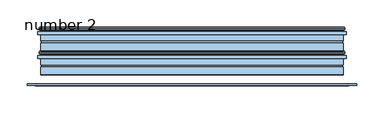
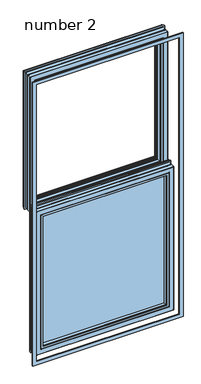
"""IFC4 building model written with IfcOpenShell, lengths in millimetres: window geometry, Window-Exterior-Sierra-Double_Hung-Operating_Unit-18inch_48inch-Width-(Hi-Divide) : number 2."""

from ifc_helpers import new_model, si_unit, frame, origin, place, context, project, spatial, polyline, ellipse_curve, outline, extrude, source, transform, mapped, element, save
from ifc_brep_helpers import plane_surface, cylinder_surface, revolved_surface, advanced_brep


def number_2_68d64fd7(model_context):
    return source(origin(), model_context, "Body", "SolidModel", [
        advanced_brep(
        [(-251.70765, 40.3779134, 2080.50765), (-251.70765, 41.5137713, 2080.50765), (251.70765, 41.5137713, 2080.50765), (251.70765, 40.3779134, 2080.50765), (-249.6812762, 41.5137713, 2078.4812762), (-249.8708265, 43.9568107, 2078.6708265), (249.8708265, 43.9568107, 2078.6708265), (249.6812762, 41.5137713, 2078.4812762), (-257.67665, 46.4921713, 2086.47665), (257.67665, 46.4921713, 2086.47665), (-257.67665, 48.8797713, 2086.47665), (257.67665, 48.8797713, 2086.47665), (-279.97785, 48.8797713, 2108.77785), (-282.36545, 46.4921713, 2111.16545), (282.36545, 46.4921713, 2111.16545), (279.97785, 48.8797713, 2108.77785), (-282.36545, 43.9267713, 2111.16545), (282.36545, 43.9267713, 2111.16545), (-280.33345, 43.9267713, 2109.13345), (-280.33345, 42.2503713, 2109.13345), (280.33345, 42.2503713, 2109.13345), (280.33345, 43.9267713, 2109.13345), (-277.03145, 42.2503713, 2105.83145), (-277.03145, 40.3453713, 2105.83145), (277.03145, 40.3453713, 2105.83145), (277.03145, 42.2503713, 2105.83145), (-284.95625, 40.3453713, 2113.75625), (-284.95625, 34.7319713, 2113.75625), (284.95625, 34.7319713, 2113.75625), (284.95625, 40.3453713, 2113.75625), (-279.64765, 34.7319713, 2108.44765), (-279.64765, 22.5399713, 2108.44765), (279.64765, 22.5399713, 2108.44765), (279.64765, 34.7319713, 2108.44765), (-279.64765, 18.5775713, 2108.44765), (279.64765, 18.5775713, 2108.44765), (-279.64765, 5.2425713, 2108.44765), (279.64765, 5.2425713, 2108.44765), (-278.83485, 4.4297713, 2107.63485), (278.83485, 4.4297713, 2107.63485), (-260.54685, 4.4297713, 2089.34685), (-260.54685, 6.3102893, 2089.34685), (260.54685, 6.3102893, 2089.34685), (260.54685, 4.4297713, 2089.34685), (-258.9459612, 6.3102893, 2087.7459612), (-258.9459612, 4.7100893, 2087.7459612), (258.9459612, 4.7100893, 2087.7459612), (258.9459612, 6.3102893, 2087.7459612), (-251.4021612, 4.7100893, 2080.2021612), (-251.4021612, 8.4780088, 2080.2021612), (251.4021612, 8.4780088, 2080.2021612), (251.4021612, 4.7100893, 2080.2021612), (-249.2398112, 8.4780088, 2078.0398112), (-248.2271612, 20.3056893, 2077.0271612), (248.2271612, 20.3056893, 2077.0271612), (249.2398112, 8.4780088, 2078.0398112), (-258.1585612, 20.3056893, 2086.9585612), (-260.54685, 17.9174005, 2089.34685), (260.54685, 17.9174005, 2089.34685), (258.1585612, 20.3056893, 2086.9585612), (-260.54685, 39.3547713, 2089.34685), (260.54685, 39.3547713, 2089.34685), (-256.9662312, 39.3547713, 2085.7662312), (-255.9430891, 40.3779134, 2084.7430891), (255.9430891, 40.3779134, 2084.7430891), (256.9662312, 39.3547713, 2085.7662312), (251.70765, 41.5137713, 1557.2486), (251.70765, 40.3779134, 1557.2486), (249.8708265, 43.9568107, 1559.0854235), (249.6812762, 41.5137713, 1559.2749738), (257.67665, 46.4921713, 1551.2796), (257.67665, 48.8797713, 1551.2796), (282.36545, 46.4921713, 1526.5908), (279.97785, 48.8797713, 1528.9784), (282.36545, 43.9267713, 1526.5908), (280.33345, 42.2503713, 1528.6228), (280.33345, 43.9267713, 1528.6228), (277.03145, 40.3453713, 1531.9248), (277.03145, 42.2503713, 1531.9248), (284.95625, 34.7319713, 1524.0), (284.95625, 40.3453713, 1524.0), (279.64765, 22.5399713, 1529.3086), (279.64765, 34.7319713, 1529.3086), (279.64765, 18.5775713, 1529.3086), (279.64765, 5.2425713, 1529.3086), (278.83485, 4.4297713, 1530.1214), (260.54685, 6.3102893, 1548.4094), (260.54685, 4.4297713, 1548.4094), (258.9459612, 4.7100893, 1550.0102888), (258.9459612, 6.3102893, 1550.0102888), (251.4021612, 8.4780088, 1557.5540888), (251.4021612, 4.7100893, 1557.5540888), (248.2271612, 20.3056893, 1560.7290888), (249.2398112, 8.4780088, 1559.7164388), (260.54685, 17.9174005, 1548.4094), (258.1585612, 20.3056893, 1550.7976888), (260.54685, 39.3547713, 1548.4094), (255.9430891, 40.3779134, 1553.0131609), (256.9662312, 39.3547713, 1551.9900188), (-251.70765, 41.5137713, 1557.2486), (-251.70765, 40.3779134, 1557.2486), (-249.8708265, 43.9568107, 1559.0854235), (-249.6812762, 41.5137713, 1559.2749738), (-257.67665, 46.4921713, 1551.2796), (-257.67665, 48.8797713, 1551.2796), (-282.36545, 46.4921713, 1526.5908), (-279.97785, 48.8797713, 1528.9784), (-282.36545, 43.9267713, 1526.5908), (-280.33345, 42.2503713, 1528.6228), (-280.33345, 43.9267713, 1528.6228), (-277.03145, 40.3453713, 1531.9248), (-277.03145, 42.2503713, 1531.9248), (-284.95625, 34.7319713, 1524.0), (-284.95625, 40.3453713, 1524.0), (-279.64765, 22.5399713, 1529.3086), (-279.64765, 34.7319713, 1529.3086), (-279.64765, 18.5775713, 1529.3086), (-279.64765, 5.2425713, 1529.3086), (-278.83485, 4.4297713, 1530.1214), (-260.54685, 6.3102893, 1548.4094), (-260.54685, 4.4297713, 1548.4094), (-258.9459612, 4.7100893, 1550.0102888), (-258.9459612, 6.3102893, 1550.0102888), (-251.4021612, 8.4780088, 1557.5540888), (-251.4021612, 4.7100893, 1557.5540888), (-248.2271612, 20.3056893, 1560.7290888), (-249.2398112, 8.4780088, 1559.7164388), (-260.54685, 17.9174005, 1548.4094), (-258.1585612, 20.3056893, 1550.7976888), (-260.54685, 39.3547713, 1548.4094), (-255.9430891, 40.3779134, 1553.0131609), (-256.9662312, 39.3547713, 1551.9900188)],
        [
            (0, 1),
            (1, 2),
            (2, 3),
            (3, 0),
            (4, 5),
            (5, 6),
            (6, 7),
            (7, 4),
            (5, 8),
            (8, 9),
            (9, 6),
            (8, 10),
            (10, 11),
            (11, 9),
            (12, 13, ellipse_curve(frame((-279.97785, 46.4921713, 2108.77785), z_axis=(0.7071067811865475, 0.0, 0.7071067811865475), x_axis=(-0.7071067811865476, 0.0, 0.7071067811865474)), 3.3765763, 2.3876)),
            (13, 14),
            (14, 15, ellipse_curve(frame((279.97785, 46.4921713, 2108.77785), z_axis=(-0.7071067811865475, 0.0, 0.7071067811865475), x_axis=(-0.7071067811865476, 0.0, -0.7071067811865474)), 3.3765763, 2.3876)),
            (15, 12),
            (13, 16),
            (16, 17),
            (17, 14),
            (18, 19),
            (19, 20),
            (20, 21),
            (21, 18),
            (22, 23),
            (23, 24),
            (24, 25),
            (25, 22),
            (26, 27),
            (27, 28),
            (28, 29),
            (29, 26),
            (30, 31),
            (31, 32),
            (32, 33),
            (33, 30),
            (31, 34, ellipse_curve(frame((-279.64765, 20.5587713, 2108.44765), z_axis=(-0.7071067811865475, 0.0, -0.7071067811865475), x_axis=(0.7071067811865476, 0.0, -0.7071067811865474)), 2.8018399, 1.9812)),
            (34, 35),
            (35, 32, ellipse_curve(frame((279.64765, 20.5587713, 2108.44765), z_axis=(0.7071067811865475, 0.0, -0.7071067811865475), x_axis=(0.7071067811865476, 0.0, 0.7071067811865474)), 2.8018399, 1.9812)),
            (34, 36),
            (36, 37),
            (37, 35),
            (36, 38, ellipse_curve(frame((-278.83485, 5.2425713, 2107.63485), z_axis=(0.7071067811865475, 0.0, 0.7071067811865475), x_axis=(-0.7071067811865476, 0.0, 0.7071067811865474)), 1.1494728, 0.8128)),
            (38, 39),
            (39, 37, ellipse_curve(frame((278.83485, 5.2425713, 2107.63485), z_axis=(-0.7071067811865475, 0.0, 0.7071067811865475), x_axis=(-0.7071067811865476, 0.0, -0.7071067811865474)), 1.1494728, 0.8128)),
            (40, 41),
            (41, 42),
            (42, 43),
            (43, 40),
            (44, 45),
            (45, 46),
            (46, 47),
            (47, 44),
            (48, 49),
            (49, 50),
            (50, 51),
            (51, 48),
            (52, 53),
            (53, 54),
            (54, 55),
            (55, 52),
            (56, 57),
            (57, 58),
            (58, 59),
            (59, 56),
            (57, 60),
            (60, 61),
            (61, 58),
            (62, 63),
            (63, 64),
            (64, 65),
            (65, 62),
            (2, 66),
            (66, 67),
            (67, 3),
            (6, 68),
            (68, 69),
            (69, 7),
            (9, 70),
            (70, 68),
            (11, 71),
            (71, 70),
            (14, 72),
            (72, 73, ellipse_curve(frame((279.97785, 46.4921713, 1528.9784), z_axis=(0.7071067811865475, 0.0, 0.7071067811865475), x_axis=(-0.7071067811865474, 0.0, 0.7071067811865476)), 3.3765763, 2.3876)),
            (73, 15),
            (17, 74),
            (74, 72),
            (20, 75),
            (75, 76),
            (76, 21),
            (24, 77),
            (77, 78),
            (78, 25),
            (28, 79),
            (79, 80),
            (80, 29),
            (32, 81),
            (81, 82),
            (82, 33),
            (35, 83),
            (83, 81, ellipse_curve(frame((279.64765, 20.5587713, 1529.3086), z_axis=(-0.7071067811865475, 0.0, -0.7071067811865475), x_axis=(0.7071067811865474, 0.0, -0.7071067811865476)), 2.8018399, 1.9812)),
            (37, 84),
            (84, 83),
            (39, 85),
            (85, 84, ellipse_curve(frame((278.83485, 5.2425713, 1530.1214), z_axis=(0.7071067811865475, 0.0, 0.7071067811865475), x_axis=(-0.7071067811865474, 0.0, 0.7071067811865476)), 1.1494728, 0.8128)),
            (42, 86),
            (86, 87),
            (87, 43),
            (46, 88),
            (88, 89),
            (89, 47),
            (50, 90),
            (90, 91),
            (91, 51),
            (54, 92),
            (92, 93),
            (93, 55),
            (58, 94),
            (94, 95),
            (95, 59),
            (61, 96),
            (96, 94),
            (64, 97),
            (97, 98),
            (98, 65),
            (66, 99),
            (99, 100),
            (100, 67),
            (68, 101),
            (101, 102),
            (102, 69),
            (70, 103),
            (103, 101),
            (71, 104),
            (104, 103),
            (72, 105),
            (105, 106, ellipse_curve(frame((-279.97785, 46.4921713, 1528.9784), z_axis=(0.7071067811865475, 0.0, -0.7071067811865475), x_axis=(0.7071067811865476, 0.0, 0.7071067811865474)), 3.3765763, 2.3876)),
            (106, 73),
            (74, 107),
            (107, 105),
            (75, 108),
            (108, 109),
            (109, 76),
            (77, 110),
            (110, 111),
            (111, 78),
            (79, 112),
            (112, 113),
            (113, 80),
            (81, 114),
            (114, 115),
            (115, 82),
            (83, 116),
            (116, 114, ellipse_curve(frame((-279.64765, 20.5587713, 1529.3086), z_axis=(-0.7071067811865475, 0.0, 0.7071067811865475), x_axis=(-0.7071067811865476, 0.0, -0.7071067811865474)), 2.8018399, 1.9812)),
            (84, 117),
            (117, 116),
            (85, 118),
            (118, 117, ellipse_curve(frame((-278.83485, 5.2425713, 1530.1214), z_axis=(0.7071067811865475, 0.0, -0.7071067811865475), x_axis=(0.7071067811865476, 0.0, 0.7071067811865474)), 1.1494728, 0.8128)),
            (86, 119),
            (119, 120),
            (120, 87),
            (88, 121),
            (121, 122),
            (122, 89),
            (90, 123),
            (123, 124),
            (124, 91),
            (92, 125),
            (125, 126),
            (126, 93),
            (94, 127),
            (127, 128),
            (128, 95),
            (96, 129),
            (129, 127),
            (97, 130),
            (130, 131),
            (131, 98),
            (63, 130),
            (100, 0),
            (99, 1),
            (102, 4),
            (101, 5),
            (103, 8),
            (104, 10),
            (106, 12),
            (105, 13),
            (107, 16),
            (109, 18),
            (108, 19),
            (111, 22),
            (110, 23),
            (113, 26),
            (112, 27),
            (115, 30),
            (114, 31),
            (116, 34),
            (117, 36),
            (118, 38),
            (120, 40),
            (119, 41),
            (122, 44),
            (121, 45),
            (124, 48),
            (123, 49),
            (126, 52),
            (125, 53),
            (128, 56),
            (127, 57),
            (129, 60),
            (131, 62),
        ],
        [
            plane_surface(frame((-251.70765, 41.5137713, 2080.50765), z_axis=(0.0, 0.0, -1.0), x_axis=(1.0, 0.0, 0.0))),
            plane_surface(frame((-249.8708265, 43.9568107, 2078.6708265), z_axis=(0.0, 0.07735544009934336, -0.9970035786731344), x_axis=(1.0, 0.0, 0.0))),
            plane_surface(frame((-257.67665, 46.4921713, 2086.47665), z_axis=(0.0, 0.9510889261909009, -0.3089172291683307), x_axis=(1.0, 0.0, 0.0))),
            plane_surface(frame((-257.67665, 48.8797713, 2086.47665), z_axis=(0.0, 0.0, -1.0), x_axis=(1.0, 0.0, 0.0))),
            cylinder_surface(frame((-284.95625, 46.4921713, 2108.77785), z_axis=(-1.0, 0.0, 0.0), x_axis=(0.0, 0.0, 1.0)), 2.3876),
            plane_surface(frame((-282.36545, 43.9267713, 2111.16545), z_axis=(0.0, 0.0, 1.0), x_axis=(1.0, 0.0, 0.0))),
            plane_surface(frame((-280.33345, 42.2503713, 2109.13345), z_axis=(0.0, 0.0, 1.0), x_axis=(1.0, 0.0, 0.0))),
            plane_surface(frame((-277.03145, 40.3453713, 2105.83145), z_axis=(0.0, 0.0, 1.0), x_axis=(1.0, 0.0, 0.0))),
            plane_surface(frame((-284.95625, 34.7319713, 2113.75625), z_axis=(0.0, 0.0, 1.0), x_axis=(1.0, 0.0, 0.0))),
            plane_surface(frame((-279.64765, 22.5399713, 2108.44765), z_axis=(0.0, 0.0, 1.0), x_axis=(1.0, 0.0, 0.0))),
            revolved_surface(polyline([(281.6288499930891, 20.5587713, 2110.4288500000002), (-281.62884999308903, 20.5587713, 2110.4288500000002)]), (-284.95625, 20.5587713, 2108.44765), (1.0, 0.0, 0.0)),
            plane_surface(frame((-279.64765, 5.2425713, 2108.44765), z_axis=(0.0, 0.0, 1.0), x_axis=(1.0, 0.0, 0.0))),
            cylinder_surface(frame((-284.95625, 5.2425713, 2107.63485), z_axis=(-1.0, 0.0, 0.0), x_axis=(0.0, 0.0, 1.0)), 0.8128),
            plane_surface(frame((-260.54685, 6.3102893, 2089.34685), z_axis=(0.0, 0.0, -1.0), x_axis=(1.0, 0.0, 0.0))),
            plane_surface(frame((-258.9459612, 4.7100893, 2087.7459612), z_axis=(0.0, 0.0, 1.0), x_axis=(1.0, 0.0, 0.0))),
            plane_surface(frame((-251.4021612, 8.4780088, 2080.2021612), z_axis=(0.0, 0.0, -1.0), x_axis=(1.0, 0.0, 0.0))),
            plane_surface(frame((-248.2271612, 20.3056893, 2077.0271612), z_axis=(0.0, -0.08530487454184653, -0.996354895797376), x_axis=(1.0, 0.0, 0.0))),
            plane_surface(frame((-260.54685, 17.9174005, 2089.34685), z_axis=(0.0, 0.7071067811865713, 0.7071067811865238), x_axis=(1.0, 0.0, 0.0))),
            plane_surface(frame((-260.54685, 39.3547713, 2089.34685), z_axis=(0.0, 0.0, -1.0), x_axis=(1.0, 0.0, 0.0))),
            plane_surface(frame((-255.9430891, 40.3779134, 2084.7430891), z_axis=(0.0, -0.7071067811861558, -0.7071067811869393), x_axis=(1.0, 0.0, 0.0))),
            plane_surface(frame((251.70765, 41.5137713, 2080.50765), z_axis=(-1.0, 0.0, 0.0), x_axis=(0.0, 0.0, -1.0))),
            plane_surface(frame((249.8708265, 43.9568107, 2078.6708265), z_axis=(-0.9970035786731344, 0.07735544009934342, 0.0), x_axis=(0.0, 0.0, -1.0))),
            plane_surface(frame((257.67665, 46.4921713, 2086.47665), z_axis=(-0.3089172291683307, 0.951088926190901, 0.0), x_axis=(0.0, 0.0, -1.0))),
            plane_surface(frame((257.67665, 48.8797713, 2086.47665), z_axis=(-1.0, 0.0, 0.0), x_axis=(0.0, 0.0, -1.0))),
            cylinder_surface(frame((279.97785, 46.4921713, 2113.75625), z_axis=(0.0, 0.0, 1.0), x_axis=(1.0, 0.0, 0.0)), 2.3876),
            plane_surface(frame((282.36545, 43.9267713, 2111.16545), z_axis=(1.0, 0.0, 0.0), x_axis=(0.0, 0.0, -1.0))),
            plane_surface(frame((280.33345, 42.2503713, 2109.13345), z_axis=(1.0, 0.0, 0.0), x_axis=(0.0, 0.0, -1.0))),
            plane_surface(frame((277.03145, 40.3453713, 2105.83145), z_axis=(1.0, 0.0, 0.0), x_axis=(0.0, 0.0, -1.0))),
            plane_surface(frame((284.95625, 34.7319713, 2113.75625), z_axis=(1.0, 0.0, 0.0), x_axis=(0.0, 0.0, -1.0))),
            plane_surface(frame((279.64765, 22.5399713, 2108.44765), z_axis=(1.0, 0.0, 0.0), x_axis=(0.0, 0.0, -1.0))),
            revolved_surface(polyline([(281.62885, 20.5587713, 1527.327400006911), (281.62885, 20.5587713, 2110.428849993089)]), (279.64765, 20.5587713, 2113.75625), (0.0, 0.0, -1.0)),
            plane_surface(frame((279.64765, 5.2425713, 2108.44765), z_axis=(1.0, 0.0, 0.0), x_axis=(0.0, 0.0, -1.0))),
            cylinder_surface(frame((278.83485, 5.2425713, 2113.75625), z_axis=(0.0, 0.0, 1.0), x_axis=(1.0, 0.0, 0.0)), 0.8128),
            plane_surface(frame((260.54685, 6.3102893, 2089.34685), z_axis=(-1.0, 0.0, 0.0), x_axis=(0.0, 0.0, -1.0))),
            plane_surface(frame((258.9459612, 4.7100893, 2087.7459612), z_axis=(1.0, 0.0, 0.0), x_axis=(0.0, 0.0, -1.0))),
            plane_surface(frame((251.4021612, 8.4780088, 2080.2021612), z_axis=(-1.0, 0.0, 0.0), x_axis=(0.0, 0.0, -1.0))),
            plane_surface(frame((248.2271612, 20.3056893, 2077.0271612), z_axis=(-0.996354895797376, -0.08530487454184647, 0.0), x_axis=(0.0, 0.0, -1.0))),
            plane_surface(frame((260.54685, 17.9174005, 2089.34685), z_axis=(0.7071067811865238, 0.7071067811865713, 0.0), x_axis=(0.0, 0.0, -1.0))),
            plane_surface(frame((260.54685, 39.3547713, 2089.34685), z_axis=(-1.0, 0.0, 0.0), x_axis=(0.0, 0.0, -1.0))),
            plane_surface(frame((255.9430891, 40.3779134, 2084.7430891), z_axis=(-0.7071067811869393, -0.7071067811861558, 0.0), x_axis=(0.0, 0.0, -1.0))),
            plane_surface(frame((251.70765, 41.5137713, 1557.2486), z_axis=(0.0, 0.0, 1.0), x_axis=(-1.0, 0.0, 0.0))),
            plane_surface(frame((249.8708265, 43.9568107, 1559.0854235), z_axis=(0.0, 0.07735544009934348, 0.9970035786731344), x_axis=(-1.0, 0.0, 0.0))),
            plane_surface(frame((257.67665, 46.4921713, 1551.2796), z_axis=(0.0, 0.951088926190901, 0.30891722916833064), x_axis=(-1.0, 0.0, 0.0))),
            plane_surface(frame((257.67665, 48.8797713, 1551.2796), z_axis=(0.0, 0.0, 1.0), x_axis=(-1.0, 0.0, 0.0))),
            cylinder_surface(frame((284.95625, 46.4921713, 1528.9784), z_axis=(1.0, 0.0, 0.0), x_axis=(0.0, 0.0, -1.0)), 2.3876),
            plane_surface(frame((282.36545, 43.9267713, 1526.5908), z_axis=(0.0, 0.0, -1.0), x_axis=(-1.0, 0.0, 0.0))),
            plane_surface(frame((280.33345, 42.2503713, 1528.6228), z_axis=(0.0, 0.0, -1.0), x_axis=(-1.0, 0.0, 0.0))),
            plane_surface(frame((277.03145, 40.3453713, 1531.9248), z_axis=(0.0, 0.0, -1.0), x_axis=(-1.0, 0.0, 0.0))),
            plane_surface(frame((284.95625, 34.7319713, 1524.0), z_axis=(0.0, 0.0, -1.0), x_axis=(-1.0, 0.0, 0.0))),
            plane_surface(frame((279.64765, 22.5399713, 1529.3086), z_axis=(0.0, 0.0, -1.0), x_axis=(-1.0, 0.0, 0.0))),
            revolved_surface(polyline([(-281.6288499930891, 20.5587713, 1527.3274000000001), (281.62884999308903, 20.5587713, 1527.3274000000001)]), (284.95625, 20.5587713, 1529.3086), (-1.0, 0.0, 0.0)),
            plane_surface(frame((279.64765, 5.2425713, 1529.3086), z_axis=(0.0, 0.0, -1.0), x_axis=(-1.0, 0.0, 0.0))),
            cylinder_surface(frame((284.95625, 5.2425713, 1530.1214), z_axis=(1.0, 0.0, 0.0), x_axis=(0.0, 0.0, -1.0)), 0.8128),
            plane_surface(frame((260.54685, 6.3102893, 1548.4094), z_axis=(0.0, 0.0, 1.0), x_axis=(-1.0, 0.0, 0.0))),
            plane_surface(frame((258.9459612, 4.7100893, 1550.0102888), z_axis=(0.0, 0.0, -1.0), x_axis=(-1.0, 0.0, 0.0))),
            plane_surface(frame((251.4021612, 8.4780088, 1557.5540888), z_axis=(0.0, 0.0, 1.0), x_axis=(-1.0, 0.0, 0.0))),
            plane_surface(frame((248.2271612, 20.3056893, 1560.7290888), z_axis=(0.0, -0.08530487454184642, 0.996354895797376), x_axis=(-1.0, 0.0, 0.0))),
            plane_surface(frame((260.54685, 17.9174005, 1548.4094), z_axis=(0.0, 0.7071067811865713, -0.7071067811865238), x_axis=(-1.0, 0.0, 0.0))),
            plane_surface(frame((260.54685, 39.3547713, 1548.4094), z_axis=(0.0, 0.0, 1.0), x_axis=(-1.0, 0.0, 0.0))),
            plane_surface(frame((255.9430891, 40.3779134, 1553.0131609), z_axis=(0.0, -0.7071067811861558, 0.7071067811869393), x_axis=(-1.0, 0.0, 0.0))),
            plane_surface(frame((-251.70765, 40.3779134, 1557.2486), z_axis=(0.0, -1.0, 0.0), x_axis=(0.0, 0.0, 1.0))),
            plane_surface(frame((-251.70765, 41.5137713, 1557.2486), z_axis=(1.0, 0.0, 0.0), x_axis=(0.0, 0.0, 1.0))),
            plane_surface(frame((-249.6812762, 41.5137713, 1559.2749738), z_axis=(0.0, -1.0, 0.0), x_axis=(0.0, 0.0, 1.0))),
            plane_surface(frame((-249.8708265, 43.9568107, 1559.0854235), z_axis=(0.9970035786731344, 0.07735544009934342, 0.0), x_axis=(0.0, 0.0, 1.0))),
            plane_surface(frame((-257.67665, 46.4921713, 1551.2796), z_axis=(0.3089172291683307, 0.951088926190901, 0.0), x_axis=(0.0, 0.0, 1.0))),
            plane_surface(frame((-257.67665, 48.8797713, 1551.2796), z_axis=(1.0, 0.0, 0.0), x_axis=(0.0, 0.0, 1.0))),
            plane_surface(frame((-279.97785, 48.8797713, 1528.9784), z_axis=(0.0, 1.0, 0.0), x_axis=(0.0, 0.0, 1.0))),
            cylinder_surface(frame((-279.97785, 46.4921713, 1524.0), z_axis=(0.0, 0.0, -1.0), x_axis=(-1.0, 0.0, 0.0)), 2.3876),
            plane_surface(frame((-282.36545, 43.9267713, 1526.5908), z_axis=(-1.0, 0.0, 0.0), x_axis=(0.0, 0.0, 1.0))),
            plane_surface(frame((-280.33345, 43.9267713, 1528.6228), z_axis=(0.0, -1.0, 0.0), x_axis=(0.0, 0.0, 1.0))),
            plane_surface(frame((-280.33345, 42.2503713, 1528.6228), z_axis=(-1.0, 0.0, 0.0), x_axis=(0.0, 0.0, 1.0))),
            plane_surface(frame((-277.03145, 42.2503713, 1531.9248), z_axis=(0.0, -1.0, 0.0), x_axis=(0.0, 0.0, 1.0))),
            plane_surface(frame((-277.03145, 40.3453713, 1531.9248), z_axis=(-1.0, 0.0, 0.0), x_axis=(0.0, 0.0, 1.0))),
            plane_surface(frame((-284.95625, 40.3453713, 1524.0), z_axis=(0.0, 1.0, 0.0), x_axis=(0.0, 0.0, 1.0))),
            plane_surface(frame((-284.95625, 34.7319713, 1524.0), z_axis=(-1.0, 0.0, 0.0), x_axis=(0.0, 0.0, 1.0))),
            plane_surface(frame((-279.64765, 34.7319713, 1529.3086), z_axis=(0.0, -1.0, 0.0), x_axis=(0.0, 0.0, 1.0))),
            plane_surface(frame((-279.64765, 22.5399713, 1529.3086), z_axis=(-1.0, 0.0, 0.0), x_axis=(0.0, 0.0, 1.0))),
            revolved_surface(polyline([(-281.62885, 20.5587713, 2110.428849993089), (-281.62885, 20.5587713, 1527.327400006911)]), (-279.64765, 20.5587713, 1524.0), (0.0, 0.0, 1.0)),
            plane_surface(frame((-279.64765, 5.2425713, 1529.3086), z_axis=(-1.0, 0.0, 0.0), x_axis=(0.0, 0.0, 1.0))),
            cylinder_surface(frame((-278.83485, 5.2425713, 1524.0), z_axis=(0.0, 0.0, -1.0), x_axis=(-1.0, 0.0, 0.0)), 0.8128),
            plane_surface(frame((-260.54685, 4.4297713, 1548.4094), z_axis=(0.0, -1.0, 0.0), x_axis=(0.0, 0.0, 1.0))),
            plane_surface(frame((-260.54685, 6.3102893, 1548.4094), z_axis=(1.0, 0.0, 0.0), x_axis=(0.0, 0.0, 1.0))),
            plane_surface(frame((-258.9459612, 6.3102893, 1550.0102888), z_axis=(0.0, -1.0, 0.0), x_axis=(0.0, 0.0, 1.0))),
            plane_surface(frame((-258.9459612, 4.7100893, 1550.0102888), z_axis=(-1.0, 0.0, 0.0), x_axis=(0.0, 0.0, 1.0))),
            plane_surface(frame((-251.4021612, 4.7100893, 1557.5540888), z_axis=(0.0, -1.0, 0.0), x_axis=(0.0, 0.0, 1.0))),
            plane_surface(frame((-251.4021612, 8.4780088, 1557.5540888), z_axis=(1.0, 0.0, 0.0), x_axis=(0.0, 0.0, 1.0))),
            plane_surface(frame((-249.2398112, 8.4780088, 1559.7164388), z_axis=(0.0, -1.0, 0.0), x_axis=(0.0, 0.0, 1.0))),
            plane_surface(frame((-248.2271612, 20.3056893, 1560.7290888), z_axis=(0.996354895797376, -0.08530487454184647, 0.0), x_axis=(0.0, 0.0, 1.0))),
            plane_surface(frame((-258.1585612, 20.3056893, 1550.7976888), z_axis=(0.0, 1.0, 0.0), x_axis=(0.0, 0.0, 1.0))),
            plane_surface(frame((-260.54685, 17.9174005, 1548.4094), z_axis=(-0.7071067811865238, 0.7071067811865713, 0.0), x_axis=(0.0, 0.0, 1.0))),
            plane_surface(frame((-260.54685, 39.3547713, 1548.4094), z_axis=(1.0, 0.0, 0.0), x_axis=(0.0, 0.0, 1.0))),
            plane_surface(frame((-256.9662312, 39.3547713, 1551.9900188), z_axis=(0.0, -1.0, 0.0), x_axis=(0.0, 0.0, 1.0))),
            plane_surface(frame((-255.9430891, 40.3779134, 1553.0131609), z_axis=(0.7071067811869393, -0.7071067811861558, 0.0), x_axis=(0.0, 0.0, 1.0))),
        ],
        [
            (0, [[1, 2, 3, 4]]),
            (1, [[5, 6, 7, 8]]),
            (2, [[9, 10, 11, -6]]),
            (3, [[12, 13, 14, -10]]),
            (4, [[15, 16, 17, 18]]),
            (5, [[19, 20, 21, -16]]),
            (6, [[22, 23, 24, 25]]),
            (7, [[26, 27, 28, 29]]),
            (8, [[30, 31, 32, 33]]),
            (9, [[34, 35, 36, 37]]),
            (10, [[38, 39, 40, -35]]),
            (11, [[41, 42, 43, -39]]),
            (12, [[44, 45, 46, -42]]),
            (13, [[47, 48, 49, 50]]),
            (14, [[51, 52, 53, 54]]),
            (15, [[55, 56, 57, 58]]),
            (16, [[59, 60, 61, 62]]),
            (17, [[63, 64, 65, 66]]),
            (18, [[67, 68, 69, -64]]),
            (19, [[70, 71, 72, 73]]),
            (20, [[-3, 74, 75, 76]]),
            (21, [[-7, 77, 78, 79]]),
            (22, [[-11, 80, 81, -77]]),
            (23, [[-14, 82, 83, -80]]),
            (24, [[-17, 84, 85, 86]]),
            (25, [[-21, 87, 88, -84]]),
            (26, [[-24, 89, 90, 91]]),
            (27, [[-28, 92, 93, 94]]),
            (28, [[-32, 95, 96, 97]]),
            (29, [[-36, 98, 99, 100]]),
            (30, [[-40, 101, 102, -98]]),
            (31, [[-43, 103, 104, -101]]),
            (32, [[-46, 105, 106, -103]]),
            (33, [[-49, 107, 108, 109]]),
            (34, [[-53, 110, 111, 112]]),
            (35, [[-57, 113, 114, 115]]),
            (36, [[-61, 116, 117, 118]]),
            (37, [[-65, 119, 120, 121]]),
            (38, [[-69, 122, 123, -119]]),
            (39, [[-72, 124, 125, 126]]),
            (40, [[-75, 127, 128, 129]]),
            (41, [[-78, 130, 131, 132]]),
            (42, [[-81, 133, 134, -130]]),
            (43, [[-83, 135, 136, -133]]),
            (44, [[-85, 137, 138, 139]]),
            (45, [[-88, 140, 141, -137]]),
            (46, [[-90, 142, 143, 144]]),
            (47, [[-93, 145, 146, 147]]),
            (48, [[-96, 148, 149, 150]]),
            (49, [[-99, 151, 152, 153]]),
            (50, [[-102, 154, 155, -151]]),
            (51, [[-104, 156, 157, -154]]),
            (52, [[-106, 158, 159, -156]]),
            (53, [[-108, 160, 161, 162]]),
            (54, [[-111, 163, 164, 165]]),
            (55, [[-114, 166, 167, 168]]),
            (56, [[-117, 169, 170, 171]]),
            (57, [[-120, 172, 173, 174]]),
            (58, [[-123, 175, 176, -172]]),
            (59, [[-125, 177, 178, 179]]),
            (60, [[180, -177, -124, -71], [-76, -129, 181, -4]]),
            (61, [[-128, 182, -1, -181]]),
            (62, [[-182, -127, -74, -2], [-79, -132, 183, -8]]),
            (63, [[-131, 184, -5, -183]]),
            (64, [[-134, 185, -9, -184]]),
            (65, [[-136, 186, -12, -185]]),
            (66, [[-86, -139, 187, -18], [-186, -135, -82, -13]]),
            (67, [[-138, 188, -15, -187]]),
            (68, [[-141, 189, -19, -188]]),
            (69, [[-189, -140, -87, -20], [-91, -144, 190, -25]]),
            (70, [[-143, 191, -22, -190]]),
            (71, [[-191, -142, -89, -23], [-94, -147, 192, -29]]),
            (72, [[-146, 193, -26, -192]]),
            (73, [[-97, -150, 194, -33], [-193, -145, -92, -27]]),
            (74, [[-149, 195, -30, -194]]),
            (75, [[-195, -148, -95, -31], [-100, -153, 196, -37]]),
            (76, [[-152, 197, -34, -196]]),
            (77, [[-155, 198, -38, -197]]),
            (78, [[-157, 199, -41, -198]]),
            (79, [[-159, 200, -44, -199]]),
            (80, [[-200, -158, -105, -45], [-109, -162, 201, -50]]),
            (81, [[-161, 202, -47, -201]]),
            (82, [[-202, -160, -107, -48], [-112, -165, 203, -54]]),
            (83, [[-164, 204, -51, -203]]),
            (84, [[-204, -163, -110, -52], [-115, -168, 205, -58]]),
            (85, [[-167, 206, -55, -205]]),
            (86, [[-206, -166, -113, -56], [-118, -171, 207, -62]]),
            (87, [[-170, 208, -59, -207]]),
            (88, [[-121, -174, 209, -66], [-208, -169, -116, -60]]),
            (89, [[-173, 210, -63, -209]]),
            (90, [[-176, 211, -67, -210]]),
            (91, [[-211, -175, -122, -68], [-126, -179, 212, -73]]),
            (92, [[-178, -180, -70, -212]]),
        ],
    ),
        extrude(outline(polyline([(-260.54685, -4.7656643), (260.54685, -4.7656643), (260.54685, -23.8147463), (-260.54685, -23.8147463), (-260.54685, -4.7656643)])), frame((0.0, 0.0, 958.65315), z_axis=(0.0, 0.0, 1.0), x_axis=(1.0, 0.0, 0.0)), (0.0, 0.0, 1.0), 570.9031),
        advanced_brep(
        [(-251.70765, -2.6066643, 967.49235), (-251.70765, -3.7425222, 967.49235), (251.70765, -3.7425222, 967.49235), (251.70765, -2.6066643, 967.49235), (-249.8708265, -0.1636249, 969.3291735), (-249.6812762, -2.6066643, 969.5187238), (249.6812762, -2.6066643, 969.5187238), (249.8708265, -0.1636249, 969.3291735), (-257.67665, 2.3717357, 961.52335), (257.67665, 2.3717357, 961.52335), (-257.67665, 4.7593357, 961.52335), (257.67665, 4.7593357, 961.52335), (-282.36545, 2.3717357, 936.83455), (-279.97785, 4.7593357, 939.22215), (279.97785, 4.7593357, 939.22215), (282.36545, 2.3717357, 936.83455), (-282.36545, -0.1936643, 936.83455), (282.36545, -0.1936643, 936.83455), (-280.33345, -1.8700643, 938.86655), (-280.33345, -0.1936643, 938.86655), (280.33345, -0.1936643, 938.86655), (280.33345, -1.8700643, 938.86655), (-277.03145, -3.7750643, 942.16855), (-277.03145, -1.8700643, 942.16855), (277.03145, -1.8700643, 942.16855), (277.03145, -3.7750643, 942.16855), (-284.95625, -9.3884643, 934.24375), (-284.95625, -3.7750643, 934.24375), (284.95625, -3.7750643, 934.24375), (284.95625, -9.3884643, 934.24375), (-279.64765, -21.5804643, 939.55235), (-279.64765, -9.3884643, 939.55235), (279.64765, -9.3884643, 939.55235), (279.64765, -21.5804643, 939.55235), (-279.64765, -25.5428643, 939.55235), (279.64765, -25.5428643, 939.55235), (-279.64765, -38.8778643, 939.55235), (279.64765, -38.8778643, 939.55235), (-278.83485, -39.6906643, 940.36515), (278.83485, -39.6906643, 940.36515), (-260.54685, -37.8101463, 958.65315), (-260.54685, -39.6906643, 958.65315), (260.54685, -39.6906643, 958.65315), (260.54685, -37.8101463, 958.65315), (-258.9459612, -39.4103463, 960.2540388), (-258.9459612, -37.8101463, 960.2540388), (258.9459612, -37.8101463, 960.2540388), (258.9459612, -39.4103463, 960.2540388), (-251.4021612, -35.6424268, 967.7978388), (-251.4021612, -39.4103463, 967.7978388), (251.4021612, -39.4103463, 967.7978388), (251.4021612, -35.6424268, 967.7978388), (-248.2271612, -23.8147463, 970.9728388), (-249.2398112, -35.6424268, 969.9601888), (249.2398112, -35.6424268, 969.9601888), (248.2271612, -23.8147463, 970.9728388), (-260.54685, -26.2030351, 958.65315), (-258.1585612, -23.8147463, 961.0414388), (258.1585612, -23.8147463, 961.0414388), (260.54685, -26.2030351, 958.65315), (-260.54685, -4.7656643, 958.65315), (260.54685, -4.7656643, 958.65315), (-255.9430891, -3.7425222, 963.2569109), (-256.9662312, -4.7656643, 962.2337688), (256.9662312, -4.7656643, 962.2337688), (255.9430891, -3.7425222, 963.2569109), (251.70765, -3.7425222, 1527.2639), (251.70765, -2.6066643, 1527.2639), (249.6812762, -2.6066643, 1525.2375262), (249.8708265, -0.1636249, 1525.4270765), (257.67665, 2.3717357, 1533.2329), (257.67665, 4.7593357, 1533.2329), (279.97785, 4.7593357, 1555.5341), (282.36545, 2.3717357, 1557.9217), (282.36545, -0.1936643, 1557.9217), (280.33345, -0.1936643, 1555.8897), (280.33345, -1.8700643, 1555.8897), (277.03145, -1.8700643, 1552.5877), (277.03145, -3.7750643, 1552.5877), (284.95625, -3.7750643, 1560.5125), (284.95625, -9.3884643, 1560.5125), (279.64765, -9.3884643, 1555.2039), (279.64765, -21.5804643, 1555.2039), (279.64765, -25.5428643, 1555.2039), (279.64765, -38.8778643, 1555.2039), (278.83485, -39.6906643, 1554.3911), (260.54685, -39.6906643, 1536.1031), (260.54685, -37.8101463, 1536.1031), (258.9459612, -37.8101463, 1534.5022112), (258.9459612, -39.4103463, 1534.5022112), (251.4021612, -39.4103463, 1526.9584112), (251.4021612, -35.6424268, 1526.9584112), (249.2398112, -35.6424268, 1524.7960612), (248.2271612, -23.8147463, 1523.7834112), (258.1585612, -23.8147463, 1533.7148112), (260.54685, -26.2030351, 1536.1031), (260.54685, -4.7656643, 1536.1031), (256.9662312, -4.7656643, 1532.5224812), (255.9430891, -3.7425222, 1531.4993391), (-251.70765, -3.7425222, 1527.2639), (-251.70765, -2.6066643, 1527.2639), (-249.6812762, -2.6066643, 1525.2375262), (-249.8708265, -0.1636249, 1525.4270765), (-257.67665, 2.3717357, 1533.2329), (-257.67665, 4.7593357, 1533.2329), (-279.97785, 4.7593357, 1555.5341), (-282.36545, 2.3717357, 1557.9217), (-282.36545, -0.1936643, 1557.9217), (-280.33345, -0.1936643, 1555.8897), (-280.33345, -1.8700643, 1555.8897), (-277.03145, -1.8700643, 1552.5877), (-277.03145, -3.7750643, 1552.5877), (-284.95625, -3.7750643, 1560.5125), (-284.95625, -9.3884643, 1560.5125), (-279.64765, -9.3884643, 1555.2039), (-279.64765, -21.5804643, 1555.2039), (-279.64765, -25.5428643, 1555.2039), (-279.64765, -38.8778643, 1555.2039), (-278.83485, -39.6906643, 1554.3911), (-260.54685, -39.6906643, 1536.1031), (-260.54685, -37.8101463, 1536.1031), (-258.9459612, -37.8101463, 1534.5022112), (-258.9459612, -39.4103463, 1534.5022112), (-251.4021612, -39.4103463, 1526.9584112), (-251.4021612, -35.6424268, 1526.9584112), (-249.2398112, -35.6424268, 1524.7960612), (-248.2271612, -23.8147463, 1523.7834112), (-258.1585612, -23.8147463, 1533.7148112), (-260.54685, -26.2030351, 1536.1031), (-260.54685, -4.7656643, 1536.1031), (-256.9662312, -4.7656643, 1532.5224812), (-255.9430891, -3.7425222, 1531.4993391)],
        [
            (0, 1),
            (1, 2),
            (2, 3),
            (3, 0),
            (4, 5),
            (5, 6),
            (6, 7),
            (7, 4),
            (8, 4),
            (7, 9),
            (9, 8),
            (10, 8),
            (9, 11),
            (11, 10),
            (12, 13, ellipse_curve(frame((-279.97785, 2.3717357, 939.22215), z_axis=(0.7071067811865475, 0.0, -0.7071067811865475), x_axis=(-0.7071067811865476, 0.0, -0.7071067811865474)), 3.3765763, 2.3876)),
            (13, 14),
            (14, 15, ellipse_curve(frame((279.97785, 2.3717357, 939.22215), z_axis=(-0.7071067811865475, 0.0, -0.7071067811865475), x_axis=(-0.7071067811865476, 0.0, 0.7071067811865474)), 3.3765763, 2.3876)),
            (15, 12),
            (16, 12),
            (15, 17),
            (17, 16),
            (18, 19),
            (19, 20),
            (20, 21),
            (21, 18),
            (22, 23),
            (23, 24),
            (24, 25),
            (25, 22),
            (26, 27),
            (27, 28),
            (28, 29),
            (29, 26),
            (30, 31),
            (31, 32),
            (32, 33),
            (33, 30),
            (34, 30, ellipse_curve(frame((-279.64765, -23.5616643, 939.55235), z_axis=(-0.7071067811865475, 0.0, 0.7071067811865475), x_axis=(0.7071067811865476, 0.0, 0.7071067811865474)), 2.8018399, 1.9812)),
            (33, 35, ellipse_curve(frame((279.64765, -23.5616643, 939.55235), z_axis=(0.7071067811865475, 0.0, 0.7071067811865475), x_axis=(0.7071067811865476, 0.0, -0.7071067811865474)), 2.8018399, 1.9812)),
            (35, 34),
            (36, 34),
            (35, 37),
            (37, 36),
            (38, 36, ellipse_curve(frame((-278.83485, -38.8778643, 940.36515), z_axis=(0.7071067811865475, 0.0, -0.7071067811865475), x_axis=(-0.7071067811865476, 0.0, -0.7071067811865474)), 1.1494728, 0.8128)),
            (37, 39, ellipse_curve(frame((278.83485, -38.8778643, 940.36515), z_axis=(-0.7071067811865475, 0.0, -0.7071067811865475), x_axis=(-0.7071067811865476, 0.0, 0.7071067811865474)), 1.1494728, 0.8128)),
            (39, 38),
            (40, 41),
            (41, 42),
            (42, 43),
            (43, 40),
            (44, 45),
            (45, 46),
            (46, 47),
            (47, 44),
            (48, 49),
            (49, 50),
            (50, 51),
            (51, 48),
            (52, 53),
            (53, 54),
            (54, 55),
            (55, 52),
            (56, 57),
            (57, 58),
            (58, 59),
            (59, 56),
            (60, 56),
            (59, 61),
            (61, 60),
            (62, 63),
            (63, 64),
            (64, 65),
            (65, 62),
            (2, 66),
            (66, 67),
            (67, 3),
            (6, 68),
            (68, 69),
            (69, 7),
            (69, 70),
            (70, 9),
            (70, 71),
            (71, 11),
            (14, 72),
            (72, 73, ellipse_curve(frame((279.97785, 2.3717357, 1555.5341), z_axis=(0.7071067811865475, 0.0, -0.7071067811865475), x_axis=(-0.7071067811865474, 0.0, -0.7071067811865476)), 3.3765763, 2.3876)),
            (73, 15),
            (73, 74),
            (74, 17),
            (20, 75),
            (75, 76),
            (76, 21),
            (24, 77),
            (77, 78),
            (78, 25),
            (28, 79),
            (79, 80),
            (80, 29),
            (32, 81),
            (81, 82),
            (82, 33),
            (82, 83, ellipse_curve(frame((279.64765, -23.5616643, 1555.2039), z_axis=(-0.7071067811865475, 0.0, 0.7071067811865475), x_axis=(0.7071067811865474, 0.0, 0.7071067811865476)), 2.8018399, 1.9812)),
            (83, 35),
            (83, 84),
            (84, 37),
            (84, 85, ellipse_curve(frame((278.83485, -38.8778643, 1554.3911), z_axis=(0.7071067811865475, 0.0, -0.7071067811865475), x_axis=(-0.7071067811865474, 0.0, -0.7071067811865476)), 1.1494728, 0.8128)),
            (85, 39),
            (42, 86),
            (86, 87),
            (87, 43),
            (46, 88),
            (88, 89),
            (89, 47),
            (50, 90),
            (90, 91),
            (91, 51),
            (54, 92),
            (92, 93),
            (93, 55),
            (58, 94),
            (94, 95),
            (95, 59),
            (95, 96),
            (96, 61),
            (64, 97),
            (97, 98),
            (98, 65),
            (66, 99),
            (99, 100),
            (100, 67),
            (68, 101),
            (101, 102),
            (102, 69),
            (102, 103),
            (103, 70),
            (103, 104),
            (104, 71),
            (72, 105),
            (105, 106, ellipse_curve(frame((-279.97785, 2.3717357, 1555.5341), z_axis=(0.7071067811865475, 0.0, 0.7071067811865475), x_axis=(0.7071067811865476, 0.0, -0.7071067811865474)), 3.3765763, 2.3876)),
            (106, 73),
            (106, 107),
            (107, 74),
            (75, 108),
            (108, 109),
            (109, 76),
            (77, 110),
            (110, 111),
            (111, 78),
            (79, 112),
            (112, 113),
            (113, 80),
            (81, 114),
            (114, 115),
            (115, 82),
            (115, 116, ellipse_curve(frame((-279.64765, -23.5616643, 1555.2039), z_axis=(-0.7071067811865475, 0.0, -0.7071067811865475), x_axis=(-0.7071067811865476, 0.0, 0.7071067811865474)), 2.8018399, 1.9812)),
            (116, 83),
            (116, 117),
            (117, 84),
            (117, 118, ellipse_curve(frame((-278.83485, -38.8778643, 1554.3911), z_axis=(0.7071067811865475, 0.0, 0.7071067811865475), x_axis=(0.7071067811865476, 0.0, -0.7071067811865474)), 1.1494728, 0.8128)),
            (118, 85),
            (86, 119),
            (119, 120),
            (120, 87),
            (88, 121),
            (121, 122),
            (122, 89),
            (90, 123),
            (123, 124),
            (124, 91),
            (92, 125),
            (125, 126),
            (126, 93),
            (94, 127),
            (127, 128),
            (128, 95),
            (128, 129),
            (129, 96),
            (97, 130),
            (130, 131),
            (131, 98),
            (131, 62),
            (1, 99),
            (0, 100),
            (5, 101),
            (4, 102),
            (8, 103),
            (10, 104),
            (13, 105),
            (12, 106),
            (16, 107),
            (19, 108),
            (18, 109),
            (23, 110),
            (22, 111),
            (27, 112),
            (26, 113),
            (31, 114),
            (30, 115),
            (34, 116),
            (36, 117),
            (38, 118),
            (41, 119),
            (40, 120),
            (45, 121),
            (44, 122),
            (49, 123),
            (48, 124),
            (53, 125),
            (52, 126),
            (57, 127),
            (56, 128),
            (60, 129),
            (63, 130),
        ],
        [
            plane_surface(frame((-251.70765, -3.7425222, 967.49235), z_axis=(0.0, 0.0, 1.0), x_axis=(1.0, 0.0, 0.0))),
            plane_surface(frame((-249.6812762, -2.6066643, 969.5187238), z_axis=(0.0, 0.07735544009934268, 0.9970035786731345), x_axis=(1.0, 0.0, 0.0))),
            plane_surface(frame((-249.8708265, -0.1636249, 969.3291735), z_axis=(0.0, 0.9510889261909015, 0.3089172291683292), x_axis=(1.0, 0.0, 0.0))),
            plane_surface(frame((-257.67665, 2.3717357, 961.52335), z_axis=(0.0, 0.0, 1.0), x_axis=(1.0, 0.0, 0.0))),
            cylinder_surface(frame((-284.95625, 2.3717357, 939.22215), z_axis=(-1.0, 0.0, 0.0), x_axis=(0.0, -1.0, 0.0)), 2.3876),
            plane_surface(frame((-282.36545, 2.3717357, 936.83455), z_axis=(0.0, 0.0, -1.0), x_axis=(1.0, 0.0, 0.0))),
            plane_surface(frame((-280.33345, -0.1936643, 938.86655), z_axis=(0.0, 0.0, -1.0), x_axis=(1.0, 0.0, 0.0))),
            plane_surface(frame((-277.03145, -1.8700643, 942.16855), z_axis=(0.0, 0.0, -1.0), x_axis=(1.0, 0.0, 0.0))),
            plane_surface(frame((-284.95625, -3.7750643, 934.24375), z_axis=(0.0, 0.0, -1.0), x_axis=(1.0, 0.0, 0.0))),
            plane_surface(frame((-279.64765, -9.3884643, 939.55235), z_axis=(0.0, 0.0, -1.0), x_axis=(1.0, 0.0, 0.0))),
            revolved_surface(polyline([(281.6288499930891, -25.5428643, 939.55235), (-281.62884999308903, -25.5428643, 939.55235)]), (-284.95625, -23.5616643, 939.55235), (1.0, 0.0, 0.0)),
            plane_surface(frame((-279.64765, -25.5428643, 939.55235), z_axis=(0.0, 0.0, -1.0), x_axis=(1.0, 0.0, 0.0))),
            cylinder_surface(frame((-284.95625, -38.8778643, 940.36515), z_axis=(-1.0, 0.0, 0.0), x_axis=(0.0, -1.0, 0.0)), 0.8128),
            plane_surface(frame((-260.54685, -39.6906643, 958.65315), z_axis=(0.0, 0.0, 1.0), x_axis=(1.0, 0.0, 0.0))),
            plane_surface(frame((-258.9459612, -37.8101463, 960.2540388), z_axis=(0.0, 0.0, -1.0), x_axis=(1.0, 0.0, 0.0))),
            plane_surface(frame((-251.4021612, -39.4103463, 967.7978388), z_axis=(0.0, 0.0, 1.0), x_axis=(1.0, 0.0, 0.0))),
            plane_surface(frame((-249.2398112, -35.6424268, 969.9601888), z_axis=(0.0, -0.08530487454184627, 0.996354895797376), x_axis=(1.0, 0.0, 0.0))),
            plane_surface(frame((-258.1585612, -23.8147463, 961.0414388), z_axis=(0.0, 0.7071067811865713, -0.7071067811865238), x_axis=(1.0, 0.0, 0.0))),
            plane_surface(frame((-260.54685, -26.2030351, 958.65315), z_axis=(0.0, 0.0, 1.0), x_axis=(1.0, 0.0, 0.0))),
            plane_surface(frame((-256.9662312, -4.7656643, 962.2337688), z_axis=(0.0, -0.7071067811861558, 0.7071067811869393), x_axis=(1.0, 0.0, 0.0))),
            plane_surface(frame((251.70765, -3.7425222, 967.49235), z_axis=(-1.0, 0.0, 0.0), x_axis=(0.0, 0.0, 1.0))),
            plane_surface(frame((249.6812762, -2.6066643, 969.5187238), z_axis=(-0.9970035786731345, 0.07735544009934263, 0.0), x_axis=(0.0, 0.0, 1.0))),
            plane_surface(frame((249.8708265, -0.1636249, 969.3291735), z_axis=(-0.30891722916832925, 0.9510889261909015, 0.0), x_axis=(0.0, 0.0, 1.0))),
            plane_surface(frame((257.67665, 2.3717357, 961.52335), z_axis=(-1.0, 0.0, 0.0), x_axis=(0.0, 0.0, 1.0))),
            cylinder_surface(frame((279.97785, 2.3717357, 934.24375), z_axis=(0.0, 0.0, -1.0), x_axis=(0.0, -1.0, 0.0)), 2.3876),
            plane_surface(frame((282.36545, 2.3717357, 936.83455), z_axis=(1.0, 0.0, 0.0), x_axis=(0.0, 0.0, 1.0))),
            plane_surface(frame((280.33345, -0.1936643, 938.86655), z_axis=(1.0, 0.0, 0.0), x_axis=(0.0, 0.0, 1.0))),
            plane_surface(frame((277.03145, -1.8700643, 942.16855), z_axis=(1.0, 0.0, 0.0), x_axis=(0.0, 0.0, 1.0))),
            plane_surface(frame((284.95625, -3.7750643, 934.24375), z_axis=(1.0, 0.0, 0.0), x_axis=(0.0, 0.0, 1.0))),
            plane_surface(frame((279.64765, -9.3884643, 939.55235), z_axis=(1.0, 0.0, 0.0), x_axis=(0.0, 0.0, 1.0))),
            revolved_surface(polyline([(279.64765, -25.5428643, 1557.185099993089), (279.64765, -25.5428643, 937.571150006911)]), (279.64765, -23.5616643, 934.24375), (0.0, 0.0, 1.0)),
            plane_surface(frame((279.64765, -25.5428643, 939.55235), z_axis=(1.0, 0.0, 0.0), x_axis=(0.0, 0.0, 1.0))),
            cylinder_surface(frame((278.83485, -38.8778643, 934.24375), z_axis=(0.0, 0.0, -1.0), x_axis=(0.0, -1.0, 0.0)), 0.8128),
            plane_surface(frame((260.54685, -39.6906643, 958.65315), z_axis=(-1.0, 0.0, 0.0), x_axis=(0.0, 0.0, 1.0))),
            plane_surface(frame((258.9459612, -37.8101463, 960.2540388), z_axis=(1.0, 0.0, 0.0), x_axis=(0.0, 0.0, 1.0))),
            plane_surface(frame((251.4021612, -39.4103463, 967.7978388), z_axis=(-1.0, 0.0, 0.0), x_axis=(0.0, 0.0, 1.0))),
            plane_surface(frame((249.2398112, -35.6424268, 969.9601888), z_axis=(-0.996354895797376, -0.08530487454184632, 0.0), x_axis=(0.0, 0.0, 1.0))),
            plane_surface(frame((258.1585612, -23.8147463, 961.0414388), z_axis=(0.7071067811865238, 0.7071067811865713, 0.0), x_axis=(0.0, 0.0, 1.0))),
            plane_surface(frame((260.54685, -26.2030351, 958.65315), z_axis=(-1.0, 0.0, 0.0), x_axis=(0.0, 0.0, 1.0))),
            plane_surface(frame((256.9662312, -4.7656643, 962.2337688), z_axis=(-0.7071067811869393, -0.7071067811861558, 0.0), x_axis=(0.0, 0.0, 1.0))),
            plane_surface(frame((251.70765, -3.7425222, 1527.2639), z_axis=(0.0, 0.0, -1.0), x_axis=(-1.0, 0.0, 0.0))),
            plane_surface(frame((249.6812762, -2.6066643, 1525.2375262), z_axis=(0.0, 0.07735544009934257, -0.9970035786731345), x_axis=(-1.0, 0.0, 0.0))),
            plane_surface(frame((249.8708265, -0.1636249, 1525.4270765), z_axis=(0.0, 0.9510889261909015, -0.3089172291683293), x_axis=(-1.0, 0.0, 0.0))),
            plane_surface(frame((257.67665, 2.3717357, 1533.2329), z_axis=(0.0, 0.0, -1.0), x_axis=(-1.0, 0.0, 0.0))),
            cylinder_surface(frame((284.95625, 2.3717357, 1555.5341), z_axis=(1.0, 0.0, 0.0), x_axis=(0.0, -1.0, 0.0)), 2.3876),
            plane_surface(frame((282.36545, 2.3717357, 1557.9217), z_axis=(0.0, 0.0, 1.0), x_axis=(-1.0, 0.0, 0.0))),
            plane_surface(frame((280.33345, -0.1936643, 1555.8897), z_axis=(0.0, 0.0, 1.0), x_axis=(-1.0, 0.0, 0.0))),
            plane_surface(frame((277.03145, -1.8700643, 1552.5877), z_axis=(0.0, 0.0, 1.0), x_axis=(-1.0, 0.0, 0.0))),
            plane_surface(frame((284.95625, -3.7750643, 1560.5125), z_axis=(0.0, 0.0, 1.0), x_axis=(-1.0, 0.0, 0.0))),
            plane_surface(frame((279.64765, -9.3884643, 1555.2039), z_axis=(0.0, 0.0, 1.0), x_axis=(-1.0, 0.0, 0.0))),
            revolved_surface(polyline([(-281.6288499930891, -25.5428643, 1555.2039), (281.62884999308903, -25.5428643, 1555.2039)]), (284.95625, -23.5616643, 1555.2039), (-1.0, 0.0, 0.0)),
            plane_surface(frame((279.64765, -25.5428643, 1555.2039), z_axis=(0.0, 0.0, 1.0), x_axis=(-1.0, 0.0, 0.0))),
            cylinder_surface(frame((284.95625, -38.8778643, 1554.3911), z_axis=(1.0, 0.0, 0.0), x_axis=(0.0, -1.0, 0.0)), 0.8128),
            plane_surface(frame((260.54685, -39.6906643, 1536.1031), z_axis=(0.0, 0.0, -1.0), x_axis=(-1.0, 0.0, 0.0))),
            plane_surface(frame((258.9459612, -37.8101463, 1534.5022112), z_axis=(0.0, 0.0, 1.0), x_axis=(-1.0, 0.0, 0.0))),
            plane_surface(frame((251.4021612, -39.4103463, 1526.9584112), z_axis=(0.0, 0.0, -1.0), x_axis=(-1.0, 0.0, 0.0))),
            plane_surface(frame((249.2398112, -35.6424268, 1524.7960612), z_axis=(0.0, -0.08530487454184638, -0.996354895797376), x_axis=(-1.0, 0.0, 0.0))),
            plane_surface(frame((258.1585612, -23.8147463, 1533.7148112), z_axis=(0.0, 0.7071067811865713, 0.7071067811865238), x_axis=(-1.0, 0.0, 0.0))),
            plane_surface(frame((260.54685, -26.2030351, 1536.1031), z_axis=(0.0, 0.0, -1.0), x_axis=(-1.0, 0.0, 0.0))),
            plane_surface(frame((256.9662312, -4.7656643, 1532.5224812), z_axis=(0.0, -0.7071067811861558, -0.7071067811869393), x_axis=(-1.0, 0.0, 0.0))),
            plane_surface(frame((-255.9430891, -3.7425222, 1531.4993391), z_axis=(0.0, -1.0, 0.0), x_axis=(0.0, 0.0, -1.0))),
            plane_surface(frame((-251.70765, -3.7425222, 1527.2639), z_axis=(1.0, 0.0, 0.0), x_axis=(0.0, 0.0, -1.0))),
            plane_surface(frame((-251.70765, -2.6066643, 1527.2639), z_axis=(0.0, -1.0, 0.0), x_axis=(0.0, 0.0, -1.0))),
            plane_surface(frame((-249.6812762, -2.6066643, 1525.2375262), z_axis=(0.9970035786731345, 0.07735544009934263, 0.0), x_axis=(0.0, 0.0, -1.0))),
            plane_surface(frame((-249.8708265, -0.1636249, 1525.4270765), z_axis=(0.30891722916832925, 0.9510889261909015, 0.0), x_axis=(0.0, 0.0, -1.0))),
            plane_surface(frame((-257.67665, 2.3717357, 1533.2329), z_axis=(1.0, 0.0, 0.0), x_axis=(0.0, 0.0, -1.0))),
            plane_surface(frame((-257.67665, 4.7593357, 1533.2329), z_axis=(0.0, 1.0, 0.0), x_axis=(0.0, 0.0, -1.0))),
            cylinder_surface(frame((-279.97785, 2.3717357, 1560.5125), z_axis=(0.0, 0.0, 1.0), x_axis=(0.0, -1.0, 0.0)), 2.3876),
            plane_surface(frame((-282.36545, 2.3717357, 1557.9217), z_axis=(-1.0, 0.0, 0.0), x_axis=(0.0, 0.0, -1.0))),
            plane_surface(frame((-282.36545, -0.1936643, 1557.9217), z_axis=(0.0, -1.0, 0.0), x_axis=(0.0, 0.0, -1.0))),
            plane_surface(frame((-280.33345, -0.1936643, 1555.8897), z_axis=(-1.0, 0.0, 0.0), x_axis=(0.0, 0.0, -1.0))),
            plane_surface(frame((-280.33345, -1.8700643, 1555.8897), z_axis=(0.0, -1.0, 0.0), x_axis=(0.0, 0.0, -1.0))),
            plane_surface(frame((-277.03145, -1.8700643, 1552.5877), z_axis=(-1.0, 0.0, 0.0), x_axis=(0.0, 0.0, -1.0))),
            plane_surface(frame((-277.03145, -3.7750643, 1552.5877), z_axis=(0.0, 1.0, 0.0), x_axis=(0.0, 0.0, -1.0))),
            plane_surface(frame((-284.95625, -3.7750643, 1560.5125), z_axis=(-1.0, 0.0, 0.0), x_axis=(0.0, 0.0, -1.0))),
            plane_surface(frame((-284.95625, -9.3884643, 1560.5125), z_axis=(0.0, -1.0, 0.0), x_axis=(0.0, 0.0, -1.0))),
            plane_surface(frame((-279.64765, -9.3884643, 1555.2039), z_axis=(-1.0, 0.0, 0.0), x_axis=(0.0, 0.0, -1.0))),
            revolved_surface(polyline([(-279.64765, -25.5428643, 937.571150006911), (-279.64765, -25.5428643, 1557.1850999930891)]), (-279.64765, -23.5616643, 1560.5125), (0.0, 0.0, -1.0)),
            plane_surface(frame((-279.64765, -25.5428643, 1555.2039), z_axis=(-1.0, 0.0, 0.0), x_axis=(0.0, 0.0, -1.0))),
            cylinder_surface(frame((-278.83485, -38.8778643, 1560.5125), z_axis=(0.0, 0.0, 1.0), x_axis=(0.0, -1.0, 0.0)), 0.8128),
            plane_surface(frame((-278.83485, -39.6906643, 1554.3911), z_axis=(0.0, -1.0, 0.0), x_axis=(0.0, 0.0, -1.0))),
            plane_surface(frame((-260.54685, -39.6906643, 1536.1031), z_axis=(1.0, 0.0, 0.0), x_axis=(0.0, 0.0, -1.0))),
            plane_surface(frame((-260.54685, -37.8101463, 1536.1031), z_axis=(0.0, -1.0, 0.0), x_axis=(0.0, 0.0, -1.0))),
            plane_surface(frame((-258.9459612, -37.8101463, 1534.5022112), z_axis=(-1.0, 0.0, 0.0), x_axis=(0.0, 0.0, -1.0))),
            plane_surface(frame((-258.9459612, -39.4103463, 1534.5022112), z_axis=(0.0, -1.0, 0.0), x_axis=(0.0, 0.0, -1.0))),
            plane_surface(frame((-251.4021612, -39.4103463, 1526.9584112), z_axis=(1.0, 0.0, 0.0), x_axis=(0.0, 0.0, -1.0))),
            plane_surface(frame((-251.4021612, -35.6424268, 1526.9584112), z_axis=(0.0, -1.0, 0.0), x_axis=(0.0, 0.0, -1.0))),
            plane_surface(frame((-249.2398112, -35.6424268, 1524.7960612), z_axis=(0.996354895797376, -0.08530487454184632, 0.0), x_axis=(0.0, 0.0, -1.0))),
            plane_surface(frame((-248.2271612, -23.8147463, 1523.7834112), z_axis=(0.0, 1.0, 0.0), x_axis=(0.0, 0.0, -1.0))),
            plane_surface(frame((-258.1585612, -23.8147463, 1533.7148112), z_axis=(-0.7071067811865238, 0.7071067811865713, 0.0), x_axis=(0.0, 0.0, -1.0))),
            plane_surface(frame((-260.54685, -26.2030351, 1536.1031), z_axis=(1.0, 0.0, 0.0), x_axis=(0.0, 0.0, -1.0))),
            plane_surface(frame((-260.54685, -4.7656643, 1536.1031), z_axis=(0.0, -1.0, 0.0), x_axis=(0.0, 0.0, -1.0))),
            plane_surface(frame((-256.9662312, -4.7656643, 1532.5224812), z_axis=(0.7071067811869393, -0.7071067811861558, 0.0), x_axis=(0.0, 0.0, -1.0))),
        ],
        [
            (0, [[1, 2, 3, 4]]),
            (1, [[5, 6, 7, 8]]),
            (2, [[9, -8, 10, 11]]),
            (3, [[12, -11, 13, 14]]),
            (4, [[15, 16, 17, 18]]),
            (5, [[19, -18, 20, 21]]),
            (6, [[22, 23, 24, 25]]),
            (7, [[26, 27, 28, 29]]),
            (8, [[30, 31, 32, 33]]),
            (9, [[34, 35, 36, 37]]),
            (10, [[38, -37, 39, 40]]),
            (11, [[41, -40, 42, 43]]),
            (12, [[44, -43, 45, 46]]),
            (13, [[47, 48, 49, 50]]),
            (14, [[51, 52, 53, 54]]),
            (15, [[55, 56, 57, 58]]),
            (16, [[59, 60, 61, 62]]),
            (17, [[63, 64, 65, 66]]),
            (18, [[67, -66, 68, 69]]),
            (19, [[70, 71, 72, 73]]),
            (20, [[-3, 74, 75, 76]]),
            (21, [[-7, 77, 78, 79]]),
            (22, [[-10, -79, 80, 81]]),
            (23, [[-13, -81, 82, 83]]),
            (24, [[-17, 84, 85, 86]]),
            (25, [[-20, -86, 87, 88]]),
            (26, [[-24, 89, 90, 91]]),
            (27, [[-28, 92, 93, 94]]),
            (28, [[-32, 95, 96, 97]]),
            (29, [[-36, 98, 99, 100]]),
            (30, [[-39, -100, 101, 102]]),
            (31, [[-42, -102, 103, 104]]),
            (32, [[-45, -104, 105, 106]]),
            (33, [[-49, 107, 108, 109]]),
            (34, [[-53, 110, 111, 112]]),
            (35, [[-57, 113, 114, 115]]),
            (36, [[-61, 116, 117, 118]]),
            (37, [[-65, 119, 120, 121]]),
            (38, [[-68, -121, 122, 123]]),
            (39, [[-72, 124, 125, 126]]),
            (40, [[-75, 127, 128, 129]]),
            (41, [[-78, 130, 131, 132]]),
            (42, [[-80, -132, 133, 134]]),
            (43, [[-82, -134, 135, 136]]),
            (44, [[-85, 137, 138, 139]]),
            (45, [[-87, -139, 140, 141]]),
            (46, [[-90, 142, 143, 144]]),
            (47, [[-93, 145, 146, 147]]),
            (48, [[-96, 148, 149, 150]]),
            (49, [[-99, 151, 152, 153]]),
            (50, [[-101, -153, 154, 155]]),
            (51, [[-103, -155, 156, 157]]),
            (52, [[-105, -157, 158, 159]]),
            (53, [[-108, 160, 161, 162]]),
            (54, [[-111, 163, 164, 165]]),
            (55, [[-114, 166, 167, 168]]),
            (56, [[-117, 169, 170, 171]]),
            (57, [[-120, 172, 173, 174]]),
            (58, [[-122, -174, 175, 176]]),
            (59, [[-125, 177, 178, 179]]),
            (60, [[-126, -179, 180, -73], [181, -127, -74, -2]]),
            (61, [[-128, -181, -1, 182]]),
            (62, [[-76, -129, -182, -4], [183, -130, -77, -6]]),
            (63, [[-131, -183, -5, 184]]),
            (64, [[-133, -184, -9, 185]]),
            (65, [[-135, -185, -12, 186]]),
            (66, [[187, -137, -84, -16], [-83, -136, -186, -14]]),
            (67, [[-138, -187, -15, 188]]),
            (68, [[-140, -188, -19, 189]]),
            (69, [[-88, -141, -189, -21], [190, -142, -89, -23]]),
            (70, [[-143, -190, -22, 191]]),
            (71, [[-91, -144, -191, -25], [192, -145, -92, -27]]),
            (72, [[-146, -192, -26, 193]]),
            (73, [[194, -148, -95, -31], [-94, -147, -193, -29]]),
            (74, [[-149, -194, -30, 195]]),
            (75, [[-97, -150, -195, -33], [196, -151, -98, -35]]),
            (76, [[-152, -196, -34, 197]]),
            (77, [[-154, -197, -38, 198]]),
            (78, [[-156, -198, -41, 199]]),
            (79, [[-158, -199, -44, 200]]),
            (80, [[-106, -159, -200, -46], [201, -160, -107, -48]]),
            (81, [[-161, -201, -47, 202]]),
            (82, [[-109, -162, -202, -50], [203, -163, -110, -52]]),
            (83, [[-164, -203, -51, 204]]),
            (84, [[-112, -165, -204, -54], [205, -166, -113, -56]]),
            (85, [[-167, -205, -55, 206]]),
            (86, [[-115, -168, -206, -58], [207, -169, -116, -60]]),
            (87, [[-170, -207, -59, 208]]),
            (88, [[209, -172, -119, -64], [-118, -171, -208, -62]]),
            (89, [[-173, -209, -63, 210]]),
            (90, [[-175, -210, -67, 211]]),
            (91, [[-123, -176, -211, -69], [212, -177, -124, -71]]),
            (92, [[-178, -212, -70, -180]]),
        ],
    ),
        extrude(outline(polyline([(2133.6, 304.8), (2133.6, -304.8), (914.4, -304.8), (914.4, 304.8), (2133.6, 304.8)]), holes=[polyline([(929.4367932, 289.7632068), (929.4367932, -289.7632068), (2118.5632068, -289.7632068), (2118.5632068, 289.7632068), (929.4367932, 289.7632068)])]), frame((0.0, -59.8487004, 0.0), z_axis=(0.0, 1.0, 0.0), x_axis=(0.0, 0.0, 1.0)), (0.0, 0.0, 1.0), 3.4924504),
    ])


if __name__ == "__main__":
    model = new_model("IFC4")
    model_context = context("Model", 3, world=origin())
    ifc_project = project(units=[si_unit("LENGTHUNIT", "METRE", prefix="MILLI")], contexts=[model_context])
    site = spatial("IfcSite", under=ifc_project)
    building = spatial("IfcBuilding", under=site)
    placement = place(None, origin())
    number_2_shape = number_2_68d64fd7(model_context)
    element("IfcWindow", 1, ObjectType="Window-Exterior-Sierra-Double_Hung-Operating_Unit-18inch_48inch-Width-(Hi-Divide) : number 2", at=placement, inside=building, context=model_context, shape_type="MappedRepresentation", body=[
        mapped(number_2_shape, transform((0.0, 0.0, 0.0), x_axis=(1.0, 0.0, 0.0), y_axis=(0.0, 1.0, 0.0), z_axis=(0.0, 0.0, 1.0))),
    ])
    save(model, "model.ifc")

# Revit data of these elements
# Type "Window-Exterior-Sierra-Double_Hung-Operating_Unit-18inch_48inch-Width-(Hi-Divide) : number 2"
#   Type Mark = "53"
#   URL = "http://www.sierrapacificwindows.com"
#   Simulite Note = "Custom Simulite Options Available"
#   Product data url = "https://bimobject.com/sierrapacificwindows/product/sierrapacificwindows_double-hung-windows"
#   Product Page URL = "http://www.sierrapacificwindows.com/double-hung-windows.cfm"
#   Product Documentation Link = "http://www.sierrapacificwindows.com/architectural/drawings/pdfs/c-dhc_16.1.pdf"
#   Model = "C-DHC-2436"
#   Manufacturer = "Sierra Pacific Windows"
#   Jamb Extension Note = "Extension Jamb may be applied on some applications. Contact your SPW sales rep. for more information"
#   Glass Type = "Insulated Glass"
#   Description = "Energy efficient, durable, and secure window"
#   Construction Type = "Wood/Clad"
#   Assembly Code = "B2030230"
#   Window Pane Thickness = 0' - 0 3/4"
#   Vertical Simulite Length = 1' - 10"
#   Thickness = 0' - 1 3/4"
#   Simulite Wood Thickness Vertical = 0' - 0 11/32"
#   Simulite Wood Thickness Horizontal = 0' - 0 13/32"
#   Simulite Width = 0' - 0 7/8"
#   Simulite Clad Thickness Vertical = 0' - 0 11/32"
#   Simulite Clad Thickness Horizontal = 0' - 0 13/32"
#   Setback = 0' - 0"
#   Rough Width = 2' - 0 3/4"
#   Rough Height = 4' - 0 3/4"
#   Interior Setback = 0' - 0"
#   Horizontal Simulite Length = 1' - 8 1/2"
#   Hi Divide Horizontal Height = 1' - 0"
#   Half Window Height = 2' - 0"
#   Frame Width = 2' - 0"
#   Height = 4' - 0"
#   Width = 2' - 0"
